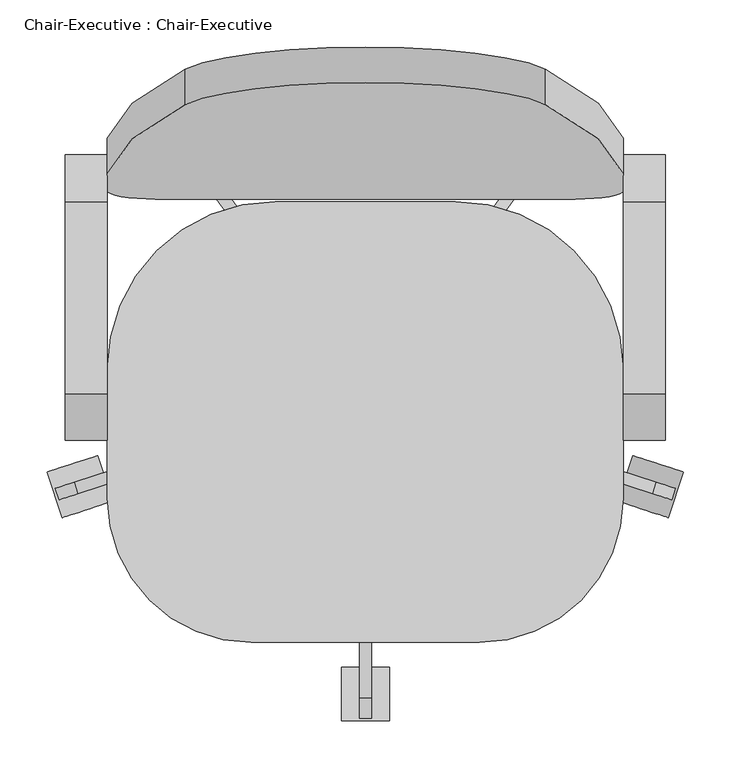
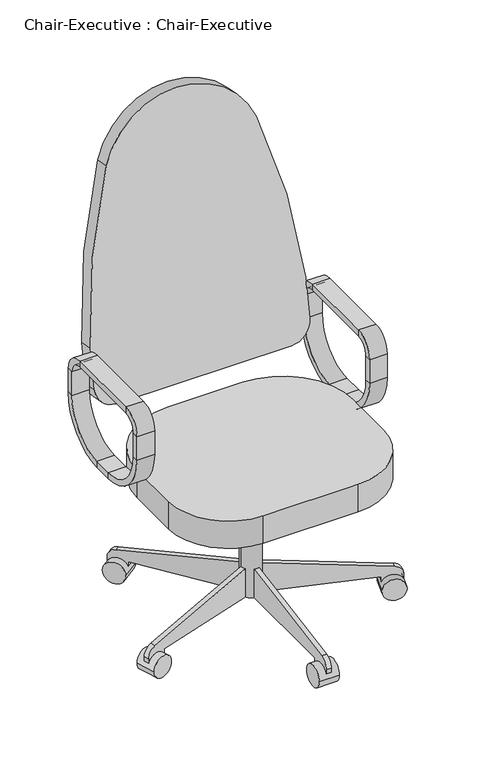
"""IFC4 building model written with IfcOpenShell, lengths in millimetres: furniture geometry, Chair-Executive : Chair-Executive."""

import ifcopenshell
import ifcopenshell.guid

model = None  # the IFC model being written
_history = None  # IfcOwnerHistory: only IFC2X3 demands one
_inside = {}  # id of a spatial element -> (the spatial element, [elements in it])
_under = {}  # id of a project, library or spatial element -> (it, [spatial elements below it])
_declared = {}  # id of a project -> (the project, [libraries it declares])
_typed = {}  # id of a type object -> (the type object, [elements of that type])
_made_of = {}  # id of a material, layer set ... -> (it, [elements and type objects made of it])


def new_model(schema):
    """Start an empty IFC model of exactly this schema.

    Asked for "IFC4X3", IfcOpenShell would pick the latest addendum, in which some entities
    have other attributes; the version numbers below select the first issue.
    IFC2X3 requires an IfcOwnerHistory on every rooted entity: one is made here for all.
    """
    global model, _history
    if schema == "IFC4X3":
        model = ifcopenshell.file(schema_version=(4, 3, 0, 0))
    else:
        model = ifcopenshell.file(schema=schema)
    _inside.clear()
    _under.clear()
    _declared.clear()
    _typed.clear()
    _made_of.clear()
    _history = None
    if model.schema == "IFC2X3":
        org = make("IfcOrganization", Name="unknown")
        user = make(
            "IfcPersonAndOrganization",
            ThePerson=make("IfcPerson", FamilyName="unknown"),
            TheOrganization=org,
        )
        app = make(
            "IfcApplication",
            ApplicationDeveloper=org,
            Version="unknown",
            ApplicationFullName="unknown",
            ApplicationIdentifier="unknown",
        )
        _history = make(
            "IfcOwnerHistory",
            OwningUser=user,
            OwningApplication=app,
            ChangeAction="ADDED",
            CreationDate=0,
        )
    return model


def make(cls, **values):
    """One entity of the class cls with the attributes given. An attribute that is None is left unset."""
    return model.create_entity(
        cls, **{name: value for name, value in values.items() if value is not None}
    )


def rooted(cls, **values):
    """An entity with a GlobalId (a new one), such as an element, a storey or a relation."""
    return make(cls, GlobalId=ifcopenshell.guid.new(), OwnerHistory=_history, **values)


def si_unit(unit_type, name, prefix=None):
    """IfcSIUnit, for example si_unit("LENGTHUNIT", "METRE", prefix="MILLI")."""
    return make("IfcSIUnit", UnitType=unit_type, Prefix=prefix, Name=name)


def assignment(units):
    """IfcUnitAssignment: the units of a project."""
    return None if units is None else make("IfcUnitAssignment", Units=units)


def point(xyz):
    """IfcCartesianPoint."""
    return None if xyz is None else make("IfcCartesianPoint", Coordinates=xyz)


def direction(xyz):
    """IfcDirection."""
    return None if xyz is None else make("IfcDirection", DirectionRatios=xyz)


def frame(location, z_axis=None, x_axis=None):
    """IfcAxis2Placement3D, a coordinate frame: its origin and axes. An axis left out is left unset."""
    return make(
        "IfcAxis2Placement3D",
        Location=point(location),
        Axis=direction(z_axis),
        RefDirection=direction(x_axis),
    )


def frame_2d(location, x_axis=None):
    """IfcAxis2Placement2D, a coordinate frame in the plane: its origin and x axis."""
    return make(
        "IfcAxis2Placement2D", Location=point(location), RefDirection=direction(x_axis)
    )


def origin():
    """The frame at (0, 0, 0) with its axes left unset."""
    return frame((0.0, 0.0, 0.0))


def place(relative_to, where):
    """IfcLocalPlacement: puts the frame where relative to a parent placement (None: the world)."""
    return make(
        "IfcLocalPlacement", PlacementRelTo=relative_to, RelativePlacement=where
    )


def context(
    kind, dimensions, precision=None, world=None, true_north=None, identifier=None
):
    """IfcGeometricRepresentationContext, for example the 3D "Model" context."""
    return make(
        "IfcGeometricRepresentationContext",
        ContextIdentifier=identifier,
        ContextType=kind,
        CoordinateSpaceDimension=dimensions,
        Precision=precision,
        WorldCoordinateSystem=world,
        TrueNorth=true_north,
    )


def project(units=None, contexts=None):
    """IfcProject with its units and contexts."""
    return rooted(
        "IfcProject",
        Name="project",
        RepresentationContexts=contexts,
        UnitsInContext=assignment(units),
    )


def spatial(cls, under=None, at=None, **own):
    """A site, building, storey or space (cls), placed at a placement, below another one or the project."""
    s = rooted(cls, ObjectPlacement=at, **own)
    if under is not None:
        _under.setdefault(under.id(), (under, []))[1].append(s)
    return s


def polyline(points):
    """IfcPolyline through the points."""
    return make("IfcPolyline", Points=[point(p) for p in points])


def circle_curve(where, radius):
    """IfcCircle in the frame where."""
    return make("IfcCircle", Position=where, Radius=radius)


def trimmed(basis, trim1, trim2, sense, master):
    """IfcTrimmedCurve: the piece of a basis curve between two trims."""
    return make(
        "IfcTrimmedCurve",
        BasisCurve=basis,
        Trim1=trim1,
        Trim2=trim2,
        SenseAgreement=sense,
        MasterRepresentation=master,
    )


def segment(curve, same_sense, transition):
    """IfcCompositeCurveSegment."""
    return make(
        "IfcCompositeCurveSegment",
        Transition=transition,
        SameSense=same_sense,
        ParentCurve=curve,
    )


def composite_curve(segments, self_intersect=None):
    """IfcCompositeCurve: segments joined end to end."""
    return make("IfcCompositeCurve", Segments=segments, SelfIntersect=self_intersect)


def outline(outer, holes=None, kind="AREA"):
    """IfcArbitraryClosedProfileDef: a profile drawn as a closed curve; with holes, ...WithVoids."""
    if holes is None:
        return make("IfcArbitraryClosedProfileDef", ProfileType=kind, OuterCurve=outer)
    return make(
        "IfcArbitraryProfileDefWithVoids",
        ProfileType=kind,
        OuterCurve=outer,
        InnerCurves=holes,
    )


def extrude(swept, where, along, depth):
    """IfcExtrudedAreaSolid: the profile swept, set in the frame where, extruded along a direction by depth."""
    return make(
        "IfcExtrudedAreaSolid",
        SweptArea=swept,
        Position=where,
        ExtrudedDirection=direction(along),
        Depth=depth,
    )


def shape(context_of_items, identifier, shape_type, items):
    """IfcShapeRepresentation: the items that make up one representation, for example the "Body"."""
    return make(
        "IfcShapeRepresentation",
        ContextOfItems=context_of_items,
        RepresentationIdentifier=identifier,
        RepresentationType=shape_type,
        Items=items,
    )


def source(mapping_origin, context_of_items, identifier, shape_type, items):
    """IfcRepresentationMap: a shape defined once, which mapped items show again and again."""
    return make(
        "IfcRepresentationMap",
        MappingOrigin=mapping_origin,
        MappedRepresentation=shape(context_of_items, identifier, shape_type, items),
    )


def transform(
    local_origin,
    x_axis=None,
    y_axis=None,
    z_axis=None,
    scale=None,
    scale2=None,
    scale3=None,
    uniform=True,
):
    """IfcCartesianTransformationOperator3D, or its non-uniform kind. x_axis, y_axis, z_axis: its Axis1, 2, 3."""
    if uniform:
        return make(
            "IfcCartesianTransformationOperator3D",
            Axis1=direction(x_axis),
            Axis2=direction(y_axis),
            LocalOrigin=point(local_origin),
            Scale=scale,
            Axis3=direction(z_axis),
        )
    return make(
        "IfcCartesianTransformationOperator3DnonUniform",
        Axis1=direction(x_axis),
        Axis2=direction(y_axis),
        LocalOrigin=point(local_origin),
        Scale=scale,
        Axis3=direction(z_axis),
        Scale2=scale2,
        Scale3=scale3,
    )


def mapped(mapping_source, mapping_target):
    """IfcMappedItem: shows the shape of a source again, moved by a transform."""
    return make(
        "IfcMappedItem", MappingSource=mapping_source, MappingTarget=mapping_target
    )


def made_of(thing, what):
    """Note that an element or type object is made of a material, layer set ...; save() writes the relation."""
    if what is not None:
        _made_of.setdefault(what.id(), (what, []))[1].append(thing)
    return thing


def element(
    cls,
    number,
    at=None,
    inside=None,
    cuts=None,
    type_object=None,
    material=None,
    context=None,
    identifier="Body",
    shape_type=None,
    held_by="IfcProductDefinitionShape",
    body=None,
    shapes=None,
    **own,
):
    """One element of the class cls, such as IfcWall. Its Tag is "e" and its number.

    at: its placement. inside: the storey or other place that contains it. cuts: it is an
    opening in that element (IfcRelVoidsElement). A single representation is given by context,
    identifier, shape_type and body (its items); several are given by shapes. held_by: the class
    of the entity that holds the representations. save() writes the other relations.
    """
    e = rooted(cls, Tag="e%d" % number, ObjectPlacement=at, **own)
    if body is not None:
        shapes = [shape(context, identifier, shape_type, body)]
    if shapes is not None:
        e.Representation = make(held_by, Representations=shapes)
    if inside is not None:
        _inside.setdefault(inside.id(), (inside, []))[1].append(e)
    if cuts is not None:
        rooted(
            "IfcRelVoidsElement", RelatingBuildingElement=cuts, RelatedOpeningElement=e
        )
    if type_object is not None:
        _typed.setdefault(type_object.id(), (type_object, []))[1].append(e)
    return made_of(e, material)


def aggregate(whole, parts):
    """IfcRelAggregates: a whole, such as a stair, and the parts it consists of."""
    return rooted("IfcRelAggregates", RelatingObject=whole, RelatedObjects=parts)


def save(model, path):
    """Write the relations noted so far, then the file.

    IfcRelAggregates (storeys below a building ...), IfcRelContainedInSpatialStructure (elements
    in a storey), IfcRelDefinesByType, IfcRelAssociatesMaterial and IfcRelDeclares: one each for
    every whole, place, type object, material and project.
    """
    for whole, parts in _under.values():
        aggregate(whole, parts)
    for where, things in _inside.values():
        rooted(
            "IfcRelContainedInSpatialStructure",
            RelatedElements=things,
            RelatingStructure=where,
        )
    for kind, things in _typed.values():
        rooted("IfcRelDefinesByType", RelatedObjects=things, RelatingType=kind)
    for what, things in _made_of.values():
        rooted("IfcRelAssociatesMaterial", RelatedObjects=things, RelatingMaterial=what)
    for by, libraries in _declared.values():
        rooted("IfcRelDeclares", RelatingContext=by, RelatedDefinitions=libraries)
    model.write(path)


def plane_surface(at):
    """IfcPlane: the flat surface through the origin of the frame at, square to its z axis."""
    return make("IfcPlane", Position=at)


def cylinder_surface(at, radius):
    """IfcCylindricalSurface: all points at the distance radius from the z axis of the frame at."""
    return make("IfcCylindricalSurface", Position=at, Radius=radius)


def revolved_surface(curve, axis_point, axis_direction):
    """IfcSurfaceOfRevolution: the curve turned about the line through axis_point along axis_direction."""
    return make(
        "IfcSurfaceOfRevolution",
        SweptCurve=make("IfcArbitraryOpenProfileDef", ProfileType="CURVE", Curve=curve),
        AxisPosition=make("IfcAxis1Placement", Location=point(axis_point), Axis=direction(axis_direction)),
    )


def advanced_brep(points, edges, surfaces, faces):
    """IfcAdvancedBrep: a solid bounded by faces that lie on surfaces and meet in shared edges.

    An edge is (start, end): straight between two places in points (the first is 0);
    or (start, end, curve); or (start, end, curve, False) where it runs against its curve.
    A face is (place in surfaces, loops), or (place, loops, False) where it looks against
    its surface's normal. A loop lists edges by number (the first is 1), with a minus sign
    where the edge is run from its end to its start. The first loop is the outer one.
    """
    corners = [point(p) for p in points]
    vertices = [make("IfcVertexPoint", VertexGeometry=c) for c in corners]
    made = []
    for start, end, *more in edges:
        made.append(
            make(
                "IfcEdgeCurve",
                EdgeStart=vertices[start],
                EdgeEnd=vertices[end],
                EdgeGeometry=more[0] if more else make("IfcPolyline", Points=[corners[start], corners[end]]),
                SameSense=more[1] if len(more) > 1 else True,
            )
        )
    hull = []
    for where, loops, *sense in faces:
        bounds = []
        for j, loop in enumerate(loops):
            ring = [make("IfcOrientedEdge", EdgeElement=made[abs(k) - 1], Orientation=k > 0) for k in loop]
            bounds.append(
                make(
                    "IfcFaceOuterBound" if j == 0 else "IfcFaceBound",
                    Bound=make("IfcEdgeLoop", EdgeList=ring),
                    Orientation=True,
                )
            )
        hull.append(make("IfcAdvancedFace", Bounds=bounds, FaceSurface=surfaces[where], SameSense=sense[0] if sense else True))
    return make("IfcAdvancedBrep", Outer=make("IfcClosedShell", CfsFaces=hull))


def chair_executive_chair_executive_a5be4872(model_context):
    return source(origin(), model_context, "Body", "SolidModel", [
        advanced_brep(
        [(-176.5091803, 217.7873012, 546.1), (-176.5091803, 233.6623012, 546.1), (-176.5091803, 108.0540984, 420.4917972), (-176.5091803, 108.0540984, 436.3667972), (-132.0591803, 217.7873012, 546.1), (-132.0591803, 108.0540984, 436.3667972), (-132.0591803, 233.6623012, 546.1), (-132.0591803, 108.0540984, 420.4917972), (-176.5091803, 217.7873012, 609.6), (-176.5091803, 233.6623012, 609.6), (-132.0591803, 217.7873012, 609.6), (-132.0591803, 233.6623012, 609.6), (-176.5091803, 184.2540984, 643.1332028), (-176.5091803, 184.2540984, 659.0082028), (-132.0591803, 184.2540984, 643.1332028), (-132.0591803, 184.2540984, 659.0082028), (-176.5091803, -18.9459016, 643.1332028), (-176.5091803, -18.9459016, 659.0082028), (-132.0591803, -18.9459016, 643.1332028), (-132.0591803, -18.9459016, 659.0082028), (-176.5091803, -52.4791044, 609.6), (-176.5091803, -68.3541044, 609.6), (-132.0591803, -52.4791044, 609.6), (-132.0591803, -68.3541044, 609.6), (-176.5091803, -52.4791044, 546.1), (-176.5091803, -68.3541044, 546.1), (-132.0591803, -52.4791044, 546.1), (-132.0591803, -68.3541044, 546.1), (-176.5091803, 57.2540984, 436.3667972), (-176.5091803, 57.2540984, 420.4917972), (-132.0591803, 57.2540984, 436.3667972), (-132.0591803, 57.2540984, 420.4917972)],
        [
            (0, 1),
            (1, 2, circle_curve(frame((-176.5091803, 108.0540984, 546.1), z_axis=(-1.0, 0.0, 0.0), x_axis=(0.0, 0.0, -1.0)), 125.6082028)),
            (2, 3),
            (3, 0, circle_curve(frame((-176.5091803, 108.0540984, 546.1), z_axis=(1.0, 0.0, 0.0), x_axis=(0.0, 0.0, -1.0)), 109.7332028)),
            (4, 0),
            (3, 5),
            (5, 4, circle_curve(frame((-132.0591803, 108.0540984, 546.1), z_axis=(1.0, 0.0, 0.0), x_axis=(0.0, 0.0, -1.0)), 109.7332028)),
            (6, 4),
            (5, 7),
            (7, 6, circle_curve(frame((-132.0591803, 108.0540984, 546.1), z_axis=(1.0, 0.0, 0.0), x_axis=(0.0, 0.0, -1.0)), 125.6082028)),
            (1, 6),
            (7, 2),
            (0, 8),
            (8, 9),
            (9, 1),
            (4, 10),
            (10, 8),
            (6, 11),
            (11, 10),
            (9, 11),
            (12, 13),
            (13, 9, circle_curve(frame((-176.5091803, 184.2540984, 609.6), z_axis=(-1.0, 0.0, 0.0), x_axis=(0.0, 1.0, 0.0)), 49.4082028)),
            (8, 12, circle_curve(frame((-176.5091803, 184.2540984, 609.6), z_axis=(1.0, 0.0, 0.0), x_axis=(0.0, 1.0, 0.0)), 33.5332028)),
            (14, 12),
            (10, 14, circle_curve(frame((-132.0591803, 184.2540984, 609.6), z_axis=(1.0, 0.0, 0.0), x_axis=(0.0, 1.0, 0.0)), 33.5332028)),
            (15, 14),
            (11, 15, circle_curve(frame((-132.0591803, 184.2540984, 609.6), z_axis=(1.0, 0.0, 0.0), x_axis=(0.0, 1.0, 0.0)), 49.4082028)),
            (13, 15),
            (12, 16),
            (16, 17),
            (17, 13),
            (14, 18),
            (18, 16),
            (15, 19),
            (19, 18),
            (17, 19),
            (20, 21),
            (21, 17, circle_curve(frame((-176.5091803, -18.9459016, 609.6), z_axis=(-1.0, 0.0, 0.0), x_axis=(0.0, 0.0, 1.0)), 49.4082028)),
            (16, 20, circle_curve(frame((-176.5091803, -18.9459016, 609.6), z_axis=(1.0, 0.0, 0.0), x_axis=(0.0, 0.0, 1.0)), 33.5332028)),
            (22, 20),
            (18, 22, circle_curve(frame((-132.0591803, -18.9459016, 609.6), z_axis=(1.0, 0.0, 0.0), x_axis=(0.0, 0.0, 1.0)), 33.5332028)),
            (23, 22),
            (19, 23, circle_curve(frame((-132.0591803, -18.9459016, 609.6), z_axis=(1.0, 0.0, 0.0), x_axis=(0.0, 0.0, 1.0)), 49.4082028)),
            (21, 23),
            (20, 24),
            (24, 25),
            (25, 21),
            (22, 26),
            (26, 24),
            (23, 27),
            (27, 26),
            (25, 27),
            (28, 29),
            (29, 25, circle_curve(frame((-176.5091803, 57.2540984, 546.1), z_axis=(-1.0, 0.0, 0.0), x_axis=(0.0, -1.0, 0.0)), 125.6082028)),
            (24, 28, circle_curve(frame((-176.5091803, 57.2540984, 546.1), z_axis=(1.0, 0.0, 0.0), x_axis=(0.0, -1.0, 0.0)), 109.7332028)),
            (30, 28),
            (26, 30, circle_curve(frame((-132.0591803, 57.2540984, 546.1), z_axis=(1.0, 0.0, 0.0), x_axis=(0.0, -1.0, 0.0)), 109.7332028)),
            (31, 30),
            (27, 31, circle_curve(frame((-132.0591803, 57.2540984, 546.1), z_axis=(1.0, 0.0, 0.0), x_axis=(0.0, -1.0, 0.0)), 125.6082028)),
            (29, 31),
            (28, 3),
            (2, 29),
            (30, 5),
            (31, 7),
        ],
        [
            plane_surface(frame((-176.5091803, 108.0540984, 546.1), z_axis=(-1.0, 0.0, 0.0), x_axis=(0.0, 0.0, -1.0))),
            revolved_surface(polyline([(-176.5091803, 108.0540984, 436.3667972), (-132.0591803, 108.0540984, 436.3667972)]), (-132.0591803, 108.0540984, 546.1), (-1.0, 0.0, 0.0)),
            plane_surface(frame((-132.0591803, 108.0540984, 546.1), z_axis=(1.0, 0.0, 0.0), x_axis=(0.0, 0.0, -1.0))),
            cylinder_surface(frame((-132.0591803, 108.0540984, 546.1), z_axis=(-1.0, 0.0, 0.0), x_axis=(0.0, 0.0, -1.0)), 125.6082028),
            plane_surface(frame((-176.5091803, 233.6623012, 546.1), z_axis=(-1.0, 0.0, 0.0), x_axis=(0.0, 0.0, 1.0))),
            plane_surface(frame((-176.5091803, 217.7873012, 546.1), z_axis=(0.0, -1.0, 0.0), x_axis=(0.0, 0.0, 1.0))),
            plane_surface(frame((-132.0591803, 217.7873012, 546.1), z_axis=(1.0, 0.0, 0.0), x_axis=(0.0, 0.0, 1.0))),
            plane_surface(frame((-132.0591803, 233.6623012, 546.1), z_axis=(0.0, 1.0, 0.0), x_axis=(0.0, 0.0, 1.0))),
            plane_surface(frame((-176.5091803, 184.2540984, 609.6), z_axis=(-1.0, 0.0, 0.0), x_axis=(0.0, 1.0, 0.0))),
            revolved_surface(polyline([(-176.5091803, 217.7873012, 609.6), (-132.0591803, 217.7873012, 609.6)]), (-132.0591803, 184.2540984, 609.6), (-1.0, 0.0, 0.0)),
            plane_surface(frame((-132.0591803, 184.2540984, 609.6), z_axis=(1.0, 0.0, 0.0), x_axis=(0.0, 1.0, 0.0))),
            cylinder_surface(frame((-132.0591803, 184.2540984, 609.6), z_axis=(-1.0, 0.0, 0.0), x_axis=(0.0, 1.0, 0.0)), 49.4082028),
            plane_surface(frame((-176.5091803, 184.2540984, 659.0082028), z_axis=(-1.0, 0.0, 0.0), x_axis=(0.0, -1.0, 0.0))),
            plane_surface(frame((-176.5091803, 184.2540984, 643.1332028), z_axis=(0.0, 0.0, -1.0), x_axis=(0.0, -1.0, 0.0))),
            plane_surface(frame((-132.0591803, 184.2540984, 643.1332028), z_axis=(1.0, 0.0, 0.0), x_axis=(0.0, -1.0, 0.0))),
            plane_surface(frame((-132.0591803, 184.2540984, 659.0082028), z_axis=(0.0, 0.0, 1.0), x_axis=(0.0, -1.0, 0.0))),
            plane_surface(frame((-176.5091803, -18.9459016, 609.6), z_axis=(-1.0, 0.0, 0.0), x_axis=(0.0, 0.0, 1.0))),
            revolved_surface(polyline([(-176.5091803, -18.9459016, 643.1332028), (-132.0591803, -18.9459016, 643.1332028)]), (-132.0591803, -18.9459016, 609.6), (-1.0, 0.0, 0.0)),
            plane_surface(frame((-132.0591803, -18.9459016, 609.6), z_axis=(1.0, 0.0, 0.0), x_axis=(0.0, 0.0, 1.0))),
            cylinder_surface(frame((-132.0591803, -18.9459016, 609.6), z_axis=(-1.0, 0.0, 0.0), x_axis=(0.0, 0.0, 1.0)), 49.4082028),
            plane_surface(frame((-176.5091803, -68.3541044, 609.6), z_axis=(-1.0, 0.0, 0.0), x_axis=(0.0, 0.0, -1.0))),
            plane_surface(frame((-176.5091803, -52.4791044, 609.6), z_axis=(0.0, 1.0, 0.0), x_axis=(0.0, 0.0, -1.0))),
            plane_surface(frame((-132.0591803, -52.4791044, 609.6), z_axis=(1.0, 0.0, 0.0), x_axis=(0.0, 0.0, -1.0))),
            plane_surface(frame((-132.0591803, -68.3541044, 609.6), z_axis=(0.0, -1.0, 0.0), x_axis=(0.0, 0.0, -1.0))),
            plane_surface(frame((-176.5091803, 57.2540984, 546.1), z_axis=(-1.0, 0.0, 0.0), x_axis=(0.0, -1.0, 0.0))),
            revolved_surface(polyline([(-176.5091803, -52.479104400000004, 546.1), (-132.0591803, -52.479104400000004, 546.1)]), (-132.0591803, 57.2540984, 546.1), (-1.0, 0.0, 0.0)),
            plane_surface(frame((-132.0591803, 57.2540984, 546.1), z_axis=(1.0, 0.0, 0.0), x_axis=(0.0, -1.0, 0.0))),
            cylinder_surface(frame((-132.0591803, 57.2540984, 546.1), z_axis=(-1.0, 0.0, 0.0), x_axis=(0.0, -1.0, 0.0)), 125.6082028),
            plane_surface(frame((-176.5091803, 57.2540984, 420.4917972), z_axis=(-1.0, 0.0, 0.0), x_axis=(0.0, 1.0, 0.0))),
            plane_surface(frame((-176.5091803, 57.2540984, 436.3667972), z_axis=(0.0, 0.0, 1.0), x_axis=(0.0, 1.0, 0.0))),
            plane_surface(frame((-132.0591803, 57.2540984, 436.3667972), z_axis=(1.0, 0.0, 0.0), x_axis=(0.0, 1.0, 0.0))),
            plane_surface(frame((-132.0591803, 57.2540984, 420.4917972), z_axis=(0.0, 0.0, -1.0), x_axis=(0.0, 1.0, 0.0))),
        ],
        [
            (0, [[1, 2, 3, 4]]),
            (1, [[5, -4, 6, 7]]),
            (2, [[8, -7, 9, 10]]),
            (3, [[11, -10, 12, -2]]),
            (4, [[13, 14, 15, -1]]),
            (5, [[16, 17, -13, -5]]),
            (6, [[18, 19, -16, -8]]),
            (7, [[-15, 20, -18, -11]]),
            (8, [[21, 22, -14, 23]]),
            (9, [[24, -23, -17, 25]]),
            (10, [[26, -25, -19, 27]]),
            (11, [[28, -27, -20, -22]]),
            (12, [[29, 30, 31, -21]]),
            (13, [[32, 33, -29, -24]]),
            (14, [[34, 35, -32, -26]]),
            (15, [[-31, 36, -34, -28]]),
            (16, [[37, 38, -30, 39]]),
            (17, [[40, -39, -33, 41]]),
            (18, [[42, -41, -35, 43]]),
            (19, [[44, -43, -36, -38]]),
            (20, [[45, 46, 47, -37]]),
            (21, [[48, 49, -45, -40]]),
            (22, [[50, 51, -48, -42]]),
            (23, [[-47, 52, -50, -44]]),
            (24, [[53, 54, -46, 55]]),
            (25, [[56, -55, -49, 57]]),
            (26, [[58, -57, -51, 59]]),
            (27, [[60, -59, -52, -54]]),
            (28, [[61, -3, 62, -53]]),
            (29, [[63, -6, -61, -56]]),
            (30, [[64, -9, -63, -58]]),
            (31, [[-62, -12, -64, -60]]),
        ],
    ),
        advanced_brep(
        [(414.0408197, 233.6623012, 546.1), (458.4908197, 233.6623012, 546.1), (458.4908197, 108.0540984, 420.4917972), (414.0408197, 108.0540984, 420.4917972), (414.0408197, 217.7873012, 546.1), (414.0408197, 108.0540984, 436.3667972), (458.4908197, 217.7873012, 546.1), (458.4908197, 108.0540984, 436.3667972), (414.0408197, 233.6623012, 609.6), (458.4908197, 233.6623012, 609.6), (414.0408197, 217.7873012, 609.6), (458.4908197, 217.7873012, 609.6), (414.0408197, 184.2540984, 659.0082028), (458.4908197, 184.2540984, 659.0082028), (414.0408197, 184.2540984, 643.1332028), (458.4908197, 184.2540984, 643.1332028), (414.0408197, -18.9459016, 659.0082028), (458.4908197, -18.9459016, 659.0082028), (414.0408197, -18.9459016, 643.1332028), (458.4908197, -18.9459016, 643.1332028), (414.0408197, -68.3541044, 609.6), (458.4908197, -68.3541044, 609.6), (414.0408197, -52.4791044, 609.6), (458.4908197, -52.4791044, 609.6), (414.0408197, -68.3541044, 546.1), (458.4908197, -68.3541044, 546.1), (414.0408197, -52.4791044, 546.1), (458.4908197, -52.4791044, 546.1), (414.0408197, 57.2540984, 420.4917972), (458.4908197, 57.2540984, 420.4917972), (414.0408197, 57.2540984, 436.3667972), (458.4908197, 57.2540984, 436.3667972)],
        [
            (0, 1),
            (1, 2, circle_curve(frame((458.4908197, 108.0540984, 546.1), z_axis=(-1.0, 0.0, 0.0), x_axis=(0.0, 0.0, -1.0)), 125.6082028)),
            (2, 3),
            (3, 0, circle_curve(frame((414.0408197, 108.0540984, 546.1), z_axis=(1.0, 0.0, 0.0), x_axis=(0.0, 0.0, -1.0)), 125.6082028)),
            (4, 0),
            (3, 5),
            (5, 4, circle_curve(frame((414.0408197, 108.0540984, 546.1), z_axis=(1.0, 0.0, 0.0), x_axis=(0.0, 0.0, -1.0)), 109.7332028)),
            (6, 4),
            (5, 7),
            (7, 6, circle_curve(frame((458.4908197, 108.0540984, 546.1), z_axis=(1.0, 0.0, 0.0), x_axis=(0.0, 0.0, -1.0)), 109.7332028)),
            (1, 6),
            (7, 2),
            (0, 8),
            (8, 9),
            (9, 1),
            (4, 10),
            (10, 8),
            (6, 11),
            (11, 10),
            (9, 11),
            (12, 13),
            (13, 9, circle_curve(frame((458.4908197, 184.2540984, 609.6), z_axis=(-1.0, 0.0, 0.0), x_axis=(0.0, 1.0, 0.0)), 49.4082028)),
            (8, 12, circle_curve(frame((414.0408197, 184.2540984, 609.6), z_axis=(1.0, 0.0, 0.0), x_axis=(0.0, 1.0, 0.0)), 49.4082028)),
            (14, 12),
            (10, 14, circle_curve(frame((414.0408197, 184.2540984, 609.6), z_axis=(1.0, 0.0, 0.0), x_axis=(0.0, 1.0, 0.0)), 33.5332028)),
            (15, 14),
            (11, 15, circle_curve(frame((458.4908197, 184.2540984, 609.6), z_axis=(1.0, 0.0, 0.0), x_axis=(0.0, 1.0, 0.0)), 33.5332028)),
            (13, 15),
            (12, 16),
            (16, 17),
            (17, 13),
            (14, 18),
            (18, 16),
            (15, 19),
            (19, 18),
            (17, 19),
            (20, 21),
            (21, 17, circle_curve(frame((458.4908197, -18.9459016, 609.6), z_axis=(-1.0, 0.0, 0.0), x_axis=(0.0, 0.0, 1.0)), 49.4082028)),
            (16, 20, circle_curve(frame((414.0408197, -18.9459016, 609.6), z_axis=(1.0, 0.0, 0.0), x_axis=(0.0, 0.0, 1.0)), 49.4082028)),
            (22, 20),
            (18, 22, circle_curve(frame((414.0408197, -18.9459016, 609.6), z_axis=(1.0, 0.0, 0.0), x_axis=(0.0, 0.0, 1.0)), 33.5332028)),
            (23, 22),
            (19, 23, circle_curve(frame((458.4908197, -18.9459016, 609.6), z_axis=(1.0, 0.0, 0.0), x_axis=(0.0, 0.0, 1.0)), 33.5332028)),
            (21, 23),
            (20, 24),
            (24, 25),
            (25, 21),
            (22, 26),
            (26, 24),
            (23, 27),
            (27, 26),
            (25, 27),
            (28, 29),
            (29, 25, circle_curve(frame((458.4908197, 57.2540984, 546.1), z_axis=(-1.0, 0.0, 0.0), x_axis=(0.0, -1.0, 0.0)), 125.6082028)),
            (24, 28, circle_curve(frame((414.0408197, 57.2540984, 546.1), z_axis=(1.0, 0.0, 0.0), x_axis=(0.0, -1.0, 0.0)), 125.6082028)),
            (30, 28),
            (26, 30, circle_curve(frame((414.0408197, 57.2540984, 546.1), z_axis=(1.0, 0.0, 0.0), x_axis=(0.0, -1.0, 0.0)), 109.7332028)),
            (31, 30),
            (27, 31, circle_curve(frame((458.4908197, 57.2540984, 546.1), z_axis=(1.0, 0.0, 0.0), x_axis=(0.0, -1.0, 0.0)), 109.7332028)),
            (29, 31),
            (28, 3),
            (2, 29),
            (30, 5),
            (31, 7),
        ],
        [
            cylinder_surface(frame((414.0408197, 108.0540984, 546.1), z_axis=(-1.0, 0.0, 0.0), x_axis=(0.0, 0.0, -1.0)), 125.6082028),
            plane_surface(frame((414.0408197, 108.0540984, 546.1), z_axis=(-1.0, 0.0, 0.0), x_axis=(0.0, 0.0, -1.0))),
            revolved_surface(polyline([(414.0408197, 108.0540984, 436.3667972), (458.4908197, 108.0540984, 436.3667972)]), (414.0408197, 108.0540984, 546.1), (-1.0, 0.0, 0.0)),
            plane_surface(frame((458.4908197, 108.0540984, 546.1), z_axis=(1.0, 0.0, 0.0), x_axis=(0.0, 0.0, -1.0))),
            plane_surface(frame((458.4908197, 233.6623012, 546.1), z_axis=(0.0, 1.0, 0.0), x_axis=(0.0, 0.0, 1.0))),
            plane_surface(frame((414.0408197, 233.6623012, 546.1), z_axis=(-1.0, 0.0, 0.0), x_axis=(0.0, 0.0, 1.0))),
            plane_surface(frame((414.0408197, 217.7873012, 546.1), z_axis=(0.0, -1.0, 0.0), x_axis=(0.0, 0.0, 1.0))),
            plane_surface(frame((458.4908197, 217.7873012, 546.1), z_axis=(1.0, 0.0, 0.0), x_axis=(0.0, 0.0, 1.0))),
            cylinder_surface(frame((414.0408197, 184.2540984, 609.6), z_axis=(-1.0, 0.0, 0.0), x_axis=(0.0, 1.0, 0.0)), 49.4082028),
            plane_surface(frame((414.0408197, 184.2540984, 609.6), z_axis=(-1.0, 0.0, 0.0), x_axis=(0.0, 1.0, 0.0))),
            revolved_surface(polyline([(414.0408197, 217.7873012, 609.6), (458.4908197, 217.7873012, 609.6)]), (414.0408197, 184.2540984, 609.6), (-1.0, 0.0, 0.0)),
            plane_surface(frame((458.4908197, 184.2540984, 609.6), z_axis=(1.0, 0.0, 0.0), x_axis=(0.0, 1.0, 0.0))),
            plane_surface(frame((458.4908197, 184.2540984, 659.0082028), z_axis=(0.0, 0.0, 1.0), x_axis=(0.0, -1.0, 0.0))),
            plane_surface(frame((414.0408197, 184.2540984, 659.0082028), z_axis=(-1.0, 0.0, 0.0), x_axis=(0.0, -1.0, 0.0))),
            plane_surface(frame((414.0408197, 184.2540984, 643.1332028), z_axis=(0.0, 0.0, -1.0), x_axis=(0.0, -1.0, 0.0))),
            plane_surface(frame((458.4908197, 184.2540984, 643.1332028), z_axis=(1.0, 0.0, 0.0), x_axis=(0.0, -1.0, 0.0))),
            cylinder_surface(frame((414.0408197, -18.9459016, 609.6), z_axis=(-1.0, 0.0, 0.0), x_axis=(0.0, 0.0, 1.0)), 49.4082028),
            plane_surface(frame((414.0408197, -18.9459016, 609.6), z_axis=(-1.0, 0.0, 0.0), x_axis=(0.0, 0.0, 1.0))),
            revolved_surface(polyline([(414.0408197, -18.9459016, 643.1332028), (458.4908197, -18.9459016, 643.1332028)]), (414.0408197, -18.9459016, 609.6), (-1.0, 0.0, 0.0)),
            plane_surface(frame((458.4908197, -18.9459016, 609.6), z_axis=(1.0, 0.0, 0.0), x_axis=(0.0, 0.0, 1.0))),
            plane_surface(frame((458.4908197, -68.3541044, 609.6), z_axis=(0.0, -1.0, 0.0), x_axis=(0.0, 0.0, -1.0))),
            plane_surface(frame((414.0408197, -68.3541044, 609.6), z_axis=(-1.0, 0.0, 0.0), x_axis=(0.0, 0.0, -1.0))),
            plane_surface(frame((414.0408197, -52.4791044, 609.6), z_axis=(0.0, 1.0, 0.0), x_axis=(0.0, 0.0, -1.0))),
            plane_surface(frame((458.4908197, -52.4791044, 609.6), z_axis=(1.0, 0.0, 0.0), x_axis=(0.0, 0.0, -1.0))),
            cylinder_surface(frame((414.0408197, 57.2540984, 546.1), z_axis=(-1.0, 0.0, 0.0), x_axis=(0.0, -1.0, 0.0)), 125.6082028),
            plane_surface(frame((414.0408197, 57.2540984, 546.1), z_axis=(-1.0, 0.0, 0.0), x_axis=(0.0, -1.0, 0.0))),
            revolved_surface(polyline([(414.0408197, -52.479104400000004, 546.1), (458.4908197, -52.479104400000004, 546.1)]), (414.0408197, 57.2540984, 546.1), (-1.0, 0.0, 0.0)),
            plane_surface(frame((458.4908197, 57.2540984, 546.1), z_axis=(1.0, 0.0, 0.0), x_axis=(0.0, -1.0, 0.0))),
            plane_surface(frame((458.4908197, 57.2540984, 420.4917972), z_axis=(0.0, 0.0, -1.0), x_axis=(0.0, 1.0, 0.0))),
            plane_surface(frame((414.0408197, 57.2540984, 420.4917972), z_axis=(-1.0, 0.0, 0.0), x_axis=(0.0, 1.0, 0.0))),
            plane_surface(frame((414.0408197, 57.2540984, 436.3667972), z_axis=(0.0, 0.0, 1.0), x_axis=(0.0, 1.0, 0.0))),
            plane_surface(frame((458.4908197, 57.2540984, 436.3667972), z_axis=(1.0, 0.0, 0.0), x_axis=(0.0, 1.0, 0.0))),
        ],
        [
            (0, [[1, 2, 3, 4]]),
            (1, [[5, -4, 6, 7]]),
            (2, [[8, -7, 9, 10]]),
            (3, [[11, -10, 12, -2]]),
            (4, [[13, 14, 15, -1]]),
            (5, [[16, 17, -13, -5]]),
            (6, [[18, 19, -16, -8]]),
            (7, [[-15, 20, -18, -11]]),
            (8, [[21, 22, -14, 23]]),
            (9, [[24, -23, -17, 25]]),
            (10, [[26, -25, -19, 27]]),
            (11, [[28, -27, -20, -22]]),
            (12, [[29, 30, 31, -21]]),
            (13, [[32, 33, -29, -24]]),
            (14, [[34, 35, -32, -26]]),
            (15, [[-31, 36, -34, -28]]),
            (16, [[37, 38, -30, 39]]),
            (17, [[40, -39, -33, 41]]),
            (18, [[42, -41, -35, 43]]),
            (19, [[44, -43, -36, -38]]),
            (20, [[45, 46, 47, -37]]),
            (21, [[48, 49, -45, -40]]),
            (22, [[50, 51, -48, -42]]),
            (23, [[-47, 52, -50, -44]]),
            (24, [[53, 54, -46, 55]]),
            (25, [[56, -55, -49, 57]]),
            (26, [[58, -57, -51, 59]]),
            (27, [[60, -59, -52, -54]]),
            (28, [[61, -3, 62, -53]]),
            (29, [[63, -6, -61, -56]]),
            (30, [[64, -9, -63, -58]]),
            (31, [[-62, -12, -64, -60]]),
        ],
    ),
        extrude(outline(composite_curve([segment(polyline([(0.0, 0.0), (-444.5, 0.0)]), True, "CONTINUOUS"), segment(trimmed(circle_curve(frame_2d((-444.5, 50.8)), 50.8), [point((-444.5, 0.0))], [point((-495.3, 50.8))], False, "CARTESIAN"), True, "CONTINUOUS"), segment(polyline([(-495.3, 50.8), (-495.3, 152.4)]), True, "CONTINUOUS"), segment(trimmed(circle_curve(frame_2d((1026.7021854, 74.3913617)), 1524.0), [point((-495.3, 152.4))], [point((-412.75, 574.9444618))], False, "CARTESIAN"), True, "CONTINUOUS"), segment(trimmed(circle_curve(frame_2d((-222.25, 504.2338544)), 203.2), [point((-412.75, 574.9444618))], [point((-31.75, 574.9444618))], False, "CARTESIAN"), True, "CONTINUOUS"), segment(trimmed(circle_curve(frame_2d((-1471.2021854, 74.3913617)), 1524.0), [point((-31.75, 574.9444618))], [point((50.8, 152.4))], False, "CARTESIAN"), True, "CONTINUOUS"), segment(polyline([(50.8, 152.4), (50.8, 50.8)]), True, "CONTINUOUS"), segment(trimmed(circle_curve(frame_2d((0.0, 50.8)), 50.8), [point((50.8, 50.8))], [point((0.0, 0.0))], False, "CARTESIAN"), True, "CONTINUOUS")], self_intersect=False)), frame((363.2408197, 224.5698964, 503.1641822), z_axis=(0.0, -0.9848077530122084, 0.17364817766692853), x_axis=(1.0, 0.0, 0.0)), (0.0, 0.0, 1.0), 38.1),
        extrude(outline(composite_curve([segment(polyline([(-132.0591803, -129.4961016), (-132.0591803, 6.4540984)]), True, "CONTINUOUS"), segment(trimmed(circle_curve(frame_2d((45.7408197, 6.4540984)), 177.8), [point((-132.0591803, 6.4540984))], [point((45.7408197, 184.2540984))], False, "CARTESIAN"), True, "CONTINUOUS"), segment(polyline([(45.7408197, 184.2540984), (236.2408197, 184.2540984)]), True, "CONTINUOUS"), segment(trimmed(circle_curve(frame_2d((236.2408197, 6.4540984)), 177.8), [point((236.2408197, 184.2540984))], [point((414.0408197, 6.4540984))], False, "CARTESIAN"), True, "CONTINUOUS"), segment(polyline([(414.0408197, 6.4540984), (414.0408197, -129.4961016)]), True, "CONTINUOUS"), segment(trimmed(circle_curve(frame_2d((261.6408197, -129.4961016)), 152.4), [point((414.0408197, -129.4961016))], [point((261.6408197, -281.8961016))], False, "CARTESIAN"), True, "CONTINUOUS"), segment(polyline([(261.6408197, -281.8961016), (20.3408197, -281.8961016)]), True, "CONTINUOUS"), segment(trimmed(circle_curve(frame_2d((20.3408197, -129.4961016)), 152.4), [point((20.3408197, -281.8961016))], [point((-132.0591803, -129.4961016))], False, "CARTESIAN"), True, "CONTINUOUS")], self_intersect=False)), frame((0.0, 0.0, 383.7835944), z_axis=(0.0, 0.0, 1.0), x_axis=(1.0, 0.0, 0.0)), (0.0, 0.0, 1.0), 73.4164056),
        extrude(outline(composite_curve([segment(trimmed(circle_curve(frame_2d((140.9908197, -18.9459016)), 25.4), [point((115.5908197, -18.9459016))], [point((166.3908197, -18.9459016))], False, "CARTESIAN"), True, "CONTINUOUS"), segment(trimmed(circle_curve(frame_2d((140.9908197, -18.9459016)), 25.4), [point((166.3908197, -18.9459016))], [point((115.5908197, -18.9459016))], False, "CARTESIAN"), True, "CONTINUOUS")], self_intersect=False)), frame((0.0, 0.0, 53.5835944), z_axis=(0.0, 0.0, 1.0), x_axis=(1.0, 0.0, 0.0)), (0.0, 0.0, 1.0), 330.5914056),
        extrude(outline(composite_curve([segment(trimmed(circle_curve(frame_2d((0.0, 28.2002728)), 28.2002727), [point((0.0, 56.4005455))], [point((0.0, 0.0))], False, "CARTESIAN"), True, "CONTINUOUS"), segment(trimmed(circle_curve(frame_2d((0.0, 28.2002728)), 28.2002727), [point((0.0, 0.0))], [point((0.0, 56.4005455))], False, "CARTESIAN"), True, "CONTINUOUS")], self_intersect=False)), frame((461.9222851, -149.9299964, 28.1835944), z_axis=(0.3090169943749423, 0.9510565162951553, 0.0), x_axis=(0.0, 0.0, -1.0)), (0.0, 0.0, 1.0), 50.8),
        extrude(outline(composite_curve([segment(polyline([(25.4, 0.0), (0.0, 0.0), (0.0, 50.8), (24.303053, 50.8)]), True, "CONTINUOUS"), segment(trimmed(circle_curve(frame_2d((24.303053, 25.4)), 25.4), [point((24.303053, 50.8))], [point((49.3171699, 29.8106636))], False, "CARTESIAN"), True, "CONTINUOUS"), segment(polyline([(49.3171699, 29.8106636), (101.6, -266.7), (101.6, -292.1), (25.4, -292.1), (25.4, 0.0)]), True, "CONTINUOUS")], self_intersect=False)), frame((416.8321702, -115.2489746, 28.1835944), z_axis=(0.3090169943749423, 0.9510565162951553, 0.0), x_axis=(0.0, 0.0, 1.0)), (0.0, 0.0, 1.0), 12.7),
        extrude(outline(composite_curve([segment(trimmed(circle_curve(frame_2d((0.0, 28.2002726)), 28.2002727), [point((0.0, 56.4005454))], [point((0.0, 0.0))], False, "CARTESIAN"), True, "CONTINUOUS"), segment(trimmed(circle_curve(frame_2d((0.0, 28.2002726)), 28.2002727), [point((0.0, 0.0))], [point((0.0, 56.4005454))], False, "CARTESIAN"), True, "CONTINUOUS")], self_intersect=False)), frame((364.7373733, 245.8017485, 28.1835944), z_axis=(-0.8090169943749499, 0.5877852522924699, 0.0), x_axis=(0.0, 0.0, -1.0)), (0.0, 0.0, 1.0), 50.8),
        extrude(outline(composite_curve([segment(polyline([(25.4, 0.0), (0.0, 0.0), (0.0, 50.8), (24.303053, 50.8)]), True, "CONTINUOUS"), segment(trimmed(circle_curve(frame_2d((24.303053, 25.3999999)), 25.4), [point((24.303053, 50.8))], [point((49.3171699, 29.8106637))], False, "CARTESIAN"), True, "CONTINUOUS"), segment(polyline([(49.3171699, 29.8106637), (101.6, -266.7), (101.6, -292.1), (25.4, -292.1), (25.4, 0.0)]), True, "CONTINUOUS")], self_intersect=False)), frame((317.8201498, 213.6355261, 28.1835944), z_axis=(-0.8090169943749499, 0.5877852522924699, 0.0), x_axis=(0.0, 0.0, 1.0)), (0.0, 0.0, 1.0), 12.7),
        extrude(outline(composite_curve([segment(trimmed(circle_curve(frame_2d((0.0, 28.2002726)), 28.2002727), [point((0.0, 56.4005454))], [point((0.0, 0.0))], False, "CARTESIAN"), True, "CONTINUOUS"), segment(trimmed(circle_curve(frame_2d((0.0, 28.2002726)), 28.2002727), [point((0.0, 0.0))], [point((0.0, 56.4005454))], False, "CARTESIAN"), True, "CONTINUOUS")], self_intersect=False)), frame((-82.755734, 245.8017485, 28.1835944), z_axis=(0.8090169943749458, 0.5877852522924754, 0.0), x_axis=(0.0, 0.0, 1.0)), (0.0, 0.0, 1.0), 50.8),
        extrude(outline(composite_curve([segment(polyline([(-25.4, 0.0), (-25.4, -292.1), (-101.6, -292.1), (-101.6, -266.6999999), (-49.3171699, 29.8106637)]), True, "CONTINUOUS"), segment(trimmed(circle_curve(frame_2d((-24.303053, 25.3999999)), 25.4), [point((-49.3171699, 29.8106637))], [point((-24.303053, 50.8))], False, "CARTESIAN"), True, "CONTINUOUS"), segment(polyline([(-24.303053, 50.8), (0.0, 50.8), (0.0, 0.0), (-25.4, 0.0)]), True, "CONTINUOUS")], self_intersect=False)), frame((-35.8385104, 213.6355261, 28.1835944), z_axis=(0.8090169943749459, 0.5877852522924754, 0.0), x_axis=(0.0, 0.0, -1.0)), (0.0, 0.0, 1.0), 12.7),
        extrude(outline(composite_curve([segment(trimmed(circle_curve(frame_2d((0.0, 28.2002727)), 28.2002727), [point((0.0, 56.4005454))], [point((0.0, 0.0))], False, "CARTESIAN"), True, "CONTINUOUS"), segment(trimmed(circle_curve(frame_2d((0.0, 28.2002727)), 28.2002727), [point((0.0, 0.0))], [point((0.0, 56.4005454))], False, "CARTESIAN"), True, "CONTINUOUS")], self_intersect=False)), frame((-179.9406457, -149.9299964, 28.1835944), z_axis=(-0.3090169943749487, 0.9510565162951532, 0.0), x_axis=(0.0, 0.0, 1.0)), (0.0, 0.0, 1.0), 50.8),
        extrude(outline(composite_curve([segment(polyline([(-25.4, 0.0), (-25.4, -292.1), (-101.6, -292.1), (-101.6, -266.7), (-49.3171699, 29.8106637)]), True, "CONTINUOUS"), segment(trimmed(circle_curve(frame_2d((-24.303053, 25.4)), 25.4), [point((-49.3171699, 29.8106637))], [point((-24.303053, 50.8000001))], False, "CARTESIAN"), True, "CONTINUOUS"), segment(polyline([(-24.303053, 50.8000001), (0.0, 50.8000001), (0.0, 0.0), (-25.4, 0.0)]), True, "CONTINUOUS")], self_intersect=False)), frame((-134.8505308, -115.2489746, 28.1835944), z_axis=(-0.3090169943749487, 0.9510565162951532, 0.0), x_axis=(0.0, 0.0, -1.0)), (0.0, 0.0, 1.0), 12.7),
        extrude(outline(composite_curve([segment(trimmed(circle_curve(frame_2d((-336.4459016, 28.1835944)), 28.2002727), [point((-308.2456289, 28.1835944))], [point((-364.6461744, 28.1835944))], False, "CARTESIAN"), True, "CONTINUOUS"), segment(trimmed(circle_curve(frame_2d((-336.4459016, 28.1835944)), 28.2002727), [point((-364.6461744, 28.1835944))], [point((-308.2456289, 28.1835944))], False, "CARTESIAN"), True, "CONTINUOUS")], self_intersect=False)), frame((115.5908197, 0.0, 0.0), z_axis=(1.0, 0.0, 0.0), x_axis=(0.0, 1.0, 0.0)), (0.0, 0.0, 1.0), 50.8),
        extrude(outline(composite_curve([segment(polyline([(-311.0459016, 53.5835944), (-311.0459016, 28.1835944), (-361.8459016, 28.1835944), (-361.8459016, 52.4866474)]), True, "CONTINUOUS"), segment(trimmed(circle_curve(frame_2d((-336.4459016, 52.4866474)), 25.4), [point((-361.8459016, 52.4866474))], [point((-340.8565654, 77.5007643))], False, "CARTESIAN"), True, "CONTINUOUS"), segment(polyline([(-340.8565654, 77.5007643), (-44.3459016, 129.7835944), (-18.9459016, 129.7835944), (-18.9459016, 53.5835944), (-311.0459016, 53.5835944)]), True, "CONTINUOUS")], self_intersect=False)), frame((134.6408197, 0.0, 0.0), z_axis=(1.0, 0.0, 0.0), x_axis=(0.0, 1.0, 0.0)), (0.0, 0.0, 1.0), 12.7),
        extrude(outline(polyline([(-69.7459016, 383.7835944), (19.1540984, 383.7835944), (19.1540984, 283.0954134), (-18.9459016, 283.0954134), (-69.7459016, 371.0835944), (-69.7459016, 383.7835944)])), frame((90.1908197, 0.0, 0.0), z_axis=(1.0, 0.0, 0.0), x_axis=(0.0, 1.0, 0.0)), (0.0, 0.0, 1.0), 101.6),
    ])


if __name__ == "__main__":
    model = new_model("IFC4")
    model_context = context("Model", 3, world=origin())
    ifc_project = project(units=[si_unit("LENGTHUNIT", "METRE", prefix="MILLI")], contexts=[model_context])
    site = spatial("IfcSite", under=ifc_project)
    building = spatial("IfcBuilding", under=site)
    placement = place(None, origin())
    chair_executive_chair_executive_shape = chair_executive_chair_executive_a5be4872(model_context)
    element("IfcFurniture", 1, ObjectType="Chair-Executive : Chair-Executive", at=placement, inside=building, context=model_context, shape_type="MappedRepresentation", body=[
        mapped(chair_executive_chair_executive_shape, transform((0.0, 0.0, 0.0), x_axis=(1.0, 0.0, 0.0), y_axis=(0.0, 1.0, 0.0), z_axis=(0.0, 0.0, 1.0))),
    ])
    save(model, "model.ifc")

# Revit data of these elements
# Type "Chair-Executive : Chair-Executive"
#   Assembly Code = "E2020200"
#   Base/Arms Material = Plastic, Opaque Black
#   Casters Material = Plastic, Opaque Black
#   Seat/Back Material = Textile - Slate Blue
#   Default Elevation = 0
# Element 1 (IfcFurniture, "Chair-Executive : Chair-Executive")
#   Materials on its faces: "Plastic, Opaque Black", "Textile - Slate Blue"
# Materials
#   "Plastic, Opaque Black": class "Plastic", colour RGB 0 0 0, transparency 0, Description = "Plastic, generic, opaque black", Cost = 0
#   "Textile - Slate Blue": class "Fabric", colour RGB 98 102 118, transparency 0
